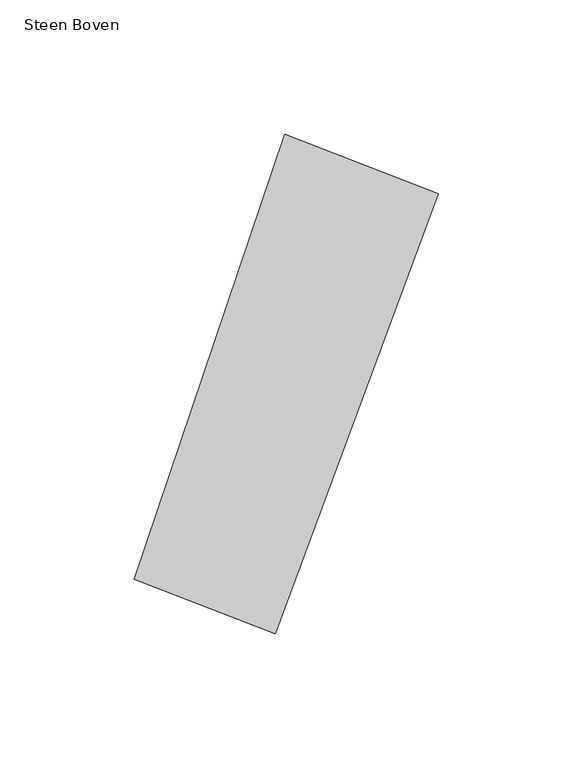
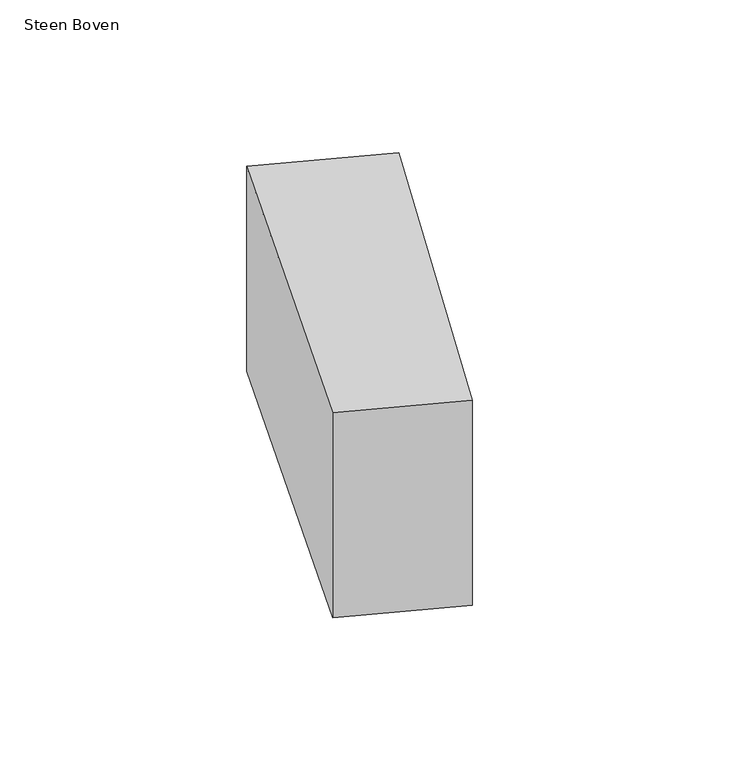
"""IFC4 building model written with IfcOpenShell, lengths in millimetres: proxy geometry, 00_GMA_steen_versie_4 : Steen Boven."""

from ifc_helpers import new_model, si_unit, origin, origin_with_axes, place, context, project, spatial, polyline, outline, extrude, source, transform, mapped, element, save


def steen_boven_9fcf3560(model_context):
    return source(origin(), model_context, "Body", "SweptSolid", [
        extrude(outline(polyline([(132.1540686, 154.8047683), (71.3620143, -9.3167174), (18.7311558, 11.0340826), (74.8608835, 176.9623931), (132.1540686, 154.8047683)])), origin_with_axes(), (0.0, 0.0, 1.0), 100.0),
    ])


if __name__ == "__main__":
    model = new_model("IFC4")
    model_context = context("Model", 3, world=origin())
    ifc_project = project(units=[si_unit("LENGTHUNIT", "METRE", prefix="MILLI")], contexts=[model_context])
    site = spatial("IfcSite", under=ifc_project)
    building = spatial("IfcBuilding", under=site)
    placement = place(None, origin())
    steen_boven_shape = steen_boven_9fcf3560(model_context)
    element("IfcBuildingElementProxy", 1, Name="00_GMA_steen_versie_4 : Steen Boven", ObjectType="00_GMA_steen_versie_4 : Steen Boven", at=placement, inside=building, context=model_context, shape_type="MappedRepresentation", body=[
        mapped(steen_boven_shape, transform((0.0, 0.0, 0.0), x_axis=(1.0, 0.0, 0.0), y_axis=(0.0, 1.0, 0.0), z_axis=(0.0, 0.0, 1.0))),
    ])
    save(model, "model.ifc")

# Revit data of these elements
# Type "00_GMA_steen_versie_4 : Steen Boven"
#   StootVoegHalfBoven [instance default] = 5 mm
#   StootVoegHalf [instance default] = 5 mm
#   StootVoegBreedteOnder = 10 mm
#   StootVoegBreedteBoven = 10 mm
#   Steendikte = 100 mm
#   LintVoegOnderHalf = 5 mm
#   LintVoegOnder = 10 mm
#   LintVoegBovenHalf = 0 mm
#   LintVoegBoven = 0 mm
#   materiaal = none
#   MateriaalVoeg = none
#   Default Elevation = 0
